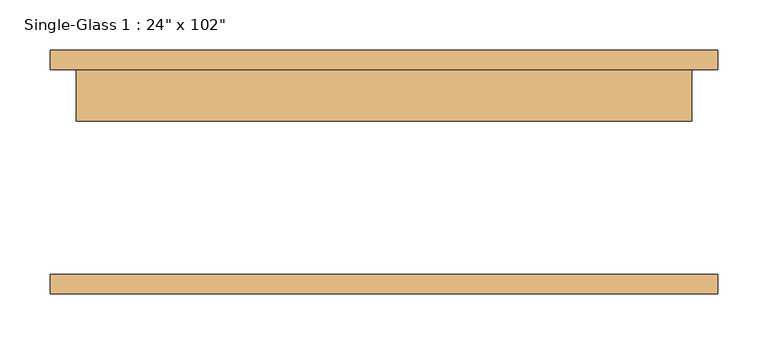
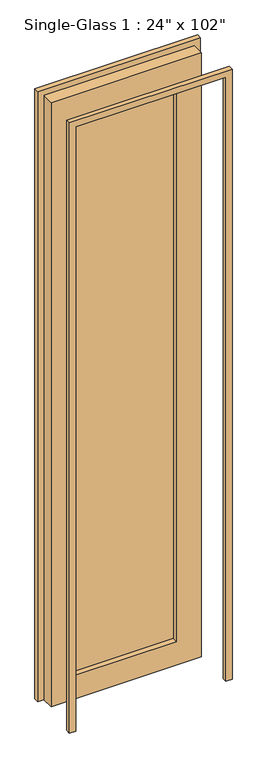
"""IFC4 building model written with IfcOpenShell, lengths in millimetres: door geometry."""

import ifcopenshell
import ifcopenshell.guid

model = None  # the IFC model being written
_history = None  # IfcOwnerHistory: only IFC2X3 demands one
_inside = {}  # id of a spatial element -> (the spatial element, [elements in it])
_under = {}  # id of a project, library or spatial element -> (it, [spatial elements below it])
_declared = {}  # id of a project -> (the project, [libraries it declares])
_typed = {}  # id of a type object -> (the type object, [elements of that type])
_made_of = {}  # id of a material, layer set ... -> (it, [elements and type objects made of it])


def new_model(schema):
    """Start an empty IFC model of exactly this schema.

    Asked for "IFC4X3", IfcOpenShell would pick the latest addendum, in which some entities
    have other attributes; the version numbers below select the first issue.
    IFC2X3 requires an IfcOwnerHistory on every rooted entity: one is made here for all.
    """
    global model, _history
    if schema == "IFC4X3":
        model = ifcopenshell.file(schema_version=(4, 3, 0, 0))
    else:
        model = ifcopenshell.file(schema=schema)
    _inside.clear()
    _under.clear()
    _declared.clear()
    _typed.clear()
    _made_of.clear()
    _history = None
    if model.schema == "IFC2X3":
        org = make("IfcOrganization", Name="unknown")
        user = make(
            "IfcPersonAndOrganization",
            ThePerson=make("IfcPerson", FamilyName="unknown"),
            TheOrganization=org,
        )
        app = make(
            "IfcApplication",
            ApplicationDeveloper=org,
            Version="unknown",
            ApplicationFullName="unknown",
            ApplicationIdentifier="unknown",
        )
        _history = make(
            "IfcOwnerHistory",
            OwningUser=user,
            OwningApplication=app,
            ChangeAction="ADDED",
            CreationDate=0,
        )
    return model


def make(cls, **values):
    """One entity of the class cls with the attributes given. An attribute that is None is left unset."""
    return model.create_entity(
        cls, **{name: value for name, value in values.items() if value is not None}
    )


def rooted(cls, **values):
    """An entity with a GlobalId (a new one), such as an element, a storey or a relation."""
    return make(cls, GlobalId=ifcopenshell.guid.new(), OwnerHistory=_history, **values)


def si_unit(unit_type, name, prefix=None):
    """IfcSIUnit, for example si_unit("LENGTHUNIT", "METRE", prefix="MILLI")."""
    return make("IfcSIUnit", UnitType=unit_type, Prefix=prefix, Name=name)


def assignment(units):
    """IfcUnitAssignment: the units of a project."""
    return None if units is None else make("IfcUnitAssignment", Units=units)


def point(xyz):
    """IfcCartesianPoint."""
    return None if xyz is None else make("IfcCartesianPoint", Coordinates=xyz)


def direction(xyz):
    """IfcDirection."""
    return None if xyz is None else make("IfcDirection", DirectionRatios=xyz)


def frame(location, z_axis=None, x_axis=None):
    """IfcAxis2Placement3D, a coordinate frame: its origin and axes. An axis left out is left unset."""
    return make(
        "IfcAxis2Placement3D",
        Location=point(location),
        Axis=direction(z_axis),
        RefDirection=direction(x_axis),
    )


def origin():
    """The frame at (0, 0, 0) with its axes left unset."""
    return frame((0.0, 0.0, 0.0))


def place(relative_to, where):
    """IfcLocalPlacement: puts the frame where relative to a parent placement (None: the world)."""
    return make(
        "IfcLocalPlacement", PlacementRelTo=relative_to, RelativePlacement=where
    )


def context(
    kind, dimensions, precision=None, world=None, true_north=None, identifier=None
):
    """IfcGeometricRepresentationContext, for example the 3D "Model" context."""
    return make(
        "IfcGeometricRepresentationContext",
        ContextIdentifier=identifier,
        ContextType=kind,
        CoordinateSpaceDimension=dimensions,
        Precision=precision,
        WorldCoordinateSystem=world,
        TrueNorth=true_north,
    )


def project(units=None, contexts=None):
    """IfcProject with its units and contexts."""
    return rooted(
        "IfcProject",
        Name="project",
        RepresentationContexts=contexts,
        UnitsInContext=assignment(units),
    )


def spatial(cls, under=None, at=None, **own):
    """A site, building, storey or space (cls), placed at a placement, below another one or the project."""
    s = rooted(cls, ObjectPlacement=at, **own)
    if under is not None:
        _under.setdefault(under.id(), (under, []))[1].append(s)
    return s


def polyline(points):
    """IfcPolyline through the points."""
    return make("IfcPolyline", Points=[point(p) for p in points])


def outline(outer, holes=None, kind="AREA"):
    """IfcArbitraryClosedProfileDef: a profile drawn as a closed curve; with holes, ...WithVoids."""
    if holes is None:
        return make("IfcArbitraryClosedProfileDef", ProfileType=kind, OuterCurve=outer)
    return make(
        "IfcArbitraryProfileDefWithVoids",
        ProfileType=kind,
        OuterCurve=outer,
        InnerCurves=holes,
    )


def extrude(swept, where, along, depth):
    """IfcExtrudedAreaSolid: the profile swept, set in the frame where, extruded along a direction by depth."""
    return make(
        "IfcExtrudedAreaSolid",
        SweptArea=swept,
        Position=where,
        ExtrudedDirection=direction(along),
        Depth=depth,
    )


def shape(context_of_items, identifier, shape_type, items):
    """IfcShapeRepresentation: the items that make up one representation, for example the "Body"."""
    return make(
        "IfcShapeRepresentation",
        ContextOfItems=context_of_items,
        RepresentationIdentifier=identifier,
        RepresentationType=shape_type,
        Items=items,
    )


def source(mapping_origin, context_of_items, identifier, shape_type, items):
    """IfcRepresentationMap: a shape defined once, which mapped items show again and again."""
    return make(
        "IfcRepresentationMap",
        MappingOrigin=mapping_origin,
        MappedRepresentation=shape(context_of_items, identifier, shape_type, items),
    )


def transform(
    local_origin,
    x_axis=None,
    y_axis=None,
    z_axis=None,
    scale=None,
    scale2=None,
    scale3=None,
    uniform=True,
):
    """IfcCartesianTransformationOperator3D, or its non-uniform kind. x_axis, y_axis, z_axis: its Axis1, 2, 3."""
    if uniform:
        return make(
            "IfcCartesianTransformationOperator3D",
            Axis1=direction(x_axis),
            Axis2=direction(y_axis),
            LocalOrigin=point(local_origin),
            Scale=scale,
            Axis3=direction(z_axis),
        )
    return make(
        "IfcCartesianTransformationOperator3DnonUniform",
        Axis1=direction(x_axis),
        Axis2=direction(y_axis),
        LocalOrigin=point(local_origin),
        Scale=scale,
        Axis3=direction(z_axis),
        Scale2=scale2,
        Scale3=scale3,
    )


def mapped(mapping_source, mapping_target):
    """IfcMappedItem: shows the shape of a source again, moved by a transform."""
    return make(
        "IfcMappedItem", MappingSource=mapping_source, MappingTarget=mapping_target
    )


def made_of(thing, what):
    """Note that an element or type object is made of a material, layer set ...; save() writes the relation."""
    if what is not None:
        _made_of.setdefault(what.id(), (what, []))[1].append(thing)
    return thing


def element(
    cls,
    number,
    at=None,
    inside=None,
    cuts=None,
    type_object=None,
    material=None,
    context=None,
    identifier="Body",
    shape_type=None,
    held_by="IfcProductDefinitionShape",
    body=None,
    shapes=None,
    **own,
):
    """One element of the class cls, such as IfcWall. Its Tag is "e" and its number.

    at: its placement. inside: the storey or other place that contains it. cuts: it is an
    opening in that element (IfcRelVoidsElement). A single representation is given by context,
    identifier, shape_type and body (its items); several are given by shapes. held_by: the class
    of the entity that holds the representations. save() writes the other relations.
    """
    e = rooted(cls, Tag="e%d" % number, ObjectPlacement=at, **own)
    if body is not None:
        shapes = [shape(context, identifier, shape_type, body)]
    if shapes is not None:
        e.Representation = make(held_by, Representations=shapes)
    if inside is not None:
        _inside.setdefault(inside.id(), (inside, []))[1].append(e)
    if cuts is not None:
        rooted(
            "IfcRelVoidsElement", RelatingBuildingElement=cuts, RelatedOpeningElement=e
        )
    if type_object is not None:
        _typed.setdefault(type_object.id(), (type_object, []))[1].append(e)
    return made_of(e, material)


def aggregate(whole, parts):
    """IfcRelAggregates: a whole, such as a stair, and the parts it consists of."""
    return rooted("IfcRelAggregates", RelatingObject=whole, RelatedObjects=parts)


def save(model, path):
    """Write the relations noted so far, then the file.

    IfcRelAggregates (storeys below a building ...), IfcRelContainedInSpatialStructure (elements
    in a storey), IfcRelDefinesByType, IfcRelAssociatesMaterial and IfcRelDeclares: one each for
    every whole, place, type object, material and project.
    """
    for whole, parts in _under.values():
        aggregate(whole, parts)
    for where, things in _inside.values():
        rooted(
            "IfcRelContainedInSpatialStructure",
            RelatedElements=things,
            RelatingStructure=where,
        )
    for kind, things in _typed.values():
        rooted("IfcRelDefinesByType", RelatedObjects=things, RelatingType=kind)
    for what, things in _made_of.values():
        rooted("IfcRelAssociatesMaterial", RelatedObjects=things, RelatingMaterial=what)
    for by, libraries in _declared.values():
        rooted("IfcRelDeclares", RelatingContext=by, RelatedDefinitions=libraries)
    model.write(path)


def door_240e8bc4(model_context):
    return source(origin(), model_context, "Body", "SweptSolid", [
        extrude(outline(polyline([(2590.8, 304.8), (0.0, 304.8), (0.0, 330.2), (2616.2, 330.2), (2616.2, -330.2), (0.0, -330.2), (0.0, -304.8), (2590.8, -304.8), (2590.8, 304.8)])), frame((0.0, -120.65, 0.0), z_axis=(0.0, 1.0, 0.0), x_axis=(0.0, 0.0, 1.0)), (0.0, 0.0, 1.0), 19.05),
        extrude(outline(polyline([(2590.8, 304.8), (0.0, 304.8), (0.0, 330.2), (2616.2, 330.2), (2616.2, -330.2), (0.0, -330.2), (0.0, -304.8), (2590.8, -304.8), (2590.8, 304.8)])), frame((0.0, 101.6, 0.0), z_axis=(0.0, 1.0, 0.0), x_axis=(0.0, 0.0, 1.0)), (0.0, 0.0, 1.0), 19.05),
        extrude(outline(polyline([(203.2, 73.025), (-203.2, 73.025), (-203.2, 79.375), (203.2, 79.375), (203.2, 73.025)])), frame((0.0, 0.0, 101.6), z_axis=(0.0, 0.0, 1.0), x_axis=(1.0, 0.0, 0.0)), (0.0, 0.0, 1.0), 2387.6),
        extrude(outline(polyline([(2590.8, 304.8), (2590.8, -304.8), (0.0, -304.8), (0.0, 304.8), (2590.8, 304.8)]), holes=[polyline([(2489.2, -203.2), (2489.2, 203.2), (101.6, 203.2), (101.6, -203.2), (2489.2, -203.2)])]), frame((0.0, 50.8, 0.0), z_axis=(0.0, 1.0, 0.0), x_axis=(0.0, 0.0, 1.0)), (0.0, 0.0, 1.0), 50.8),
    ])


if __name__ == "__main__":
    model = new_model("IFC4")
    model_context = context("Model", 3, world=origin())
    ifc_project = project(units=[si_unit("LENGTHUNIT", "METRE", prefix="MILLI")], contexts=[model_context])
    site = spatial("IfcSite", under=ifc_project)
    building = spatial("IfcBuilding", under=site)
    placement = place(None, origin())
    door_shape = door_240e8bc4(model_context)
    element("IfcDoor", 1, ObjectType="Single-Glass 1 : 24\" x 102\"", at=placement, inside=building, context=model_context, shape_type="MappedRepresentation", body=[
        mapped(door_shape, transform((0.0, 0.0, 0.0), x_axis=(1.0, 0.0, 0.0), y_axis=(0.0, 1.0, 0.0), z_axis=(0.0, 0.0, 1.0))),
    ])
    save(model, "model.ifc")

# Revit data of these elements
# Type "Single-Glass 1 : 24\" x 102\""
#   Type Mark = "35"
#   Assembly Code = "C1020"
#   Thickness = 0' - 2"
#   Height = 8' - 6"
#   Rail Width - Base = 0' - 4"
#   Rail Width - Top = 0' - 4"
#   Stile Width - Hinge = 0' - 4"
#   Stile Width - Latch = 0' - 4"
#   Trim Projection Ext = 0' - 0 3/4"
#   Trim Projection Int = 0' - 0 3/4"
#   Trim Width = 0' - 1"
#   Width = 2' - 0"
#   Door Material = Door - Panel
#   Frame Material = Door - Frame
#   Function = (empty or 0)
#   Wall Closure = (empty or 0)
# Element 1 (IfcDoor, "Single-Glass 1 : 24\" x 102\"")
#   Materials on its faces: "Door - Frame", "Door - Panel", "Glass"
# Materials
#   "Door - Panel": class "Wood", colour RGB 210 159 95, transparency 0
#   "Door - Frame": class "Miscellaneous", colour RGB 118 70 51, transparency 0
#   "Glass": class "Glass", colour RGB 0 128 192, transparency 0.75
